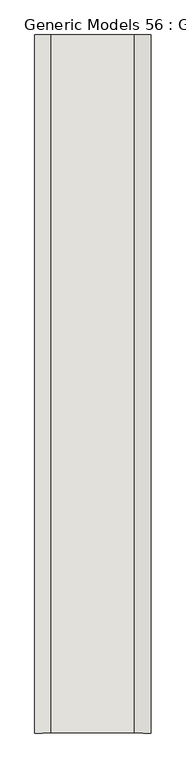
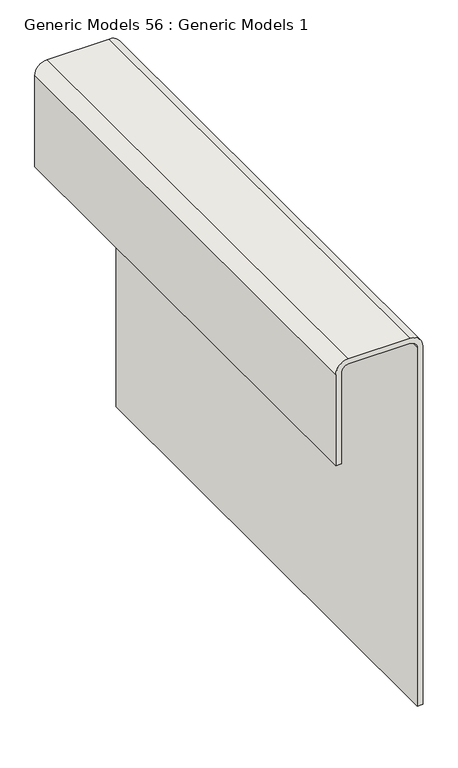
"""IFC4 building model written with IfcOpenShell, lengths in millimetres: wall geometry, Generic Models 56 : Generic Models 1."""

import ifcopenshell
import ifcopenshell.guid

model = None  # the IFC model being written
_history = None  # IfcOwnerHistory: only IFC2X3 demands one
_inside = {}  # id of a spatial element -> (the spatial element, [elements in it])
_under = {}  # id of a project, library or spatial element -> (it, [spatial elements below it])
_declared = {}  # id of a project -> (the project, [libraries it declares])
_typed = {}  # id of a type object -> (the type object, [elements of that type])
_made_of = {}  # id of a material, layer set ... -> (it, [elements and type objects made of it])


def new_model(schema):
    """Start an empty IFC model of exactly this schema.

    Asked for "IFC4X3", IfcOpenShell would pick the latest addendum, in which some entities
    have other attributes; the version numbers below select the first issue.
    IFC2X3 requires an IfcOwnerHistory on every rooted entity: one is made here for all.
    """
    global model, _history
    if schema == "IFC4X3":
        model = ifcopenshell.file(schema_version=(4, 3, 0, 0))
    else:
        model = ifcopenshell.file(schema=schema)
    _inside.clear()
    _under.clear()
    _declared.clear()
    _typed.clear()
    _made_of.clear()
    _history = None
    if model.schema == "IFC2X3":
        org = make("IfcOrganization", Name="unknown")
        user = make(
            "IfcPersonAndOrganization",
            ThePerson=make("IfcPerson", FamilyName="unknown"),
            TheOrganization=org,
        )
        app = make(
            "IfcApplication",
            ApplicationDeveloper=org,
            Version="unknown",
            ApplicationFullName="unknown",
            ApplicationIdentifier="unknown",
        )
        _history = make(
            "IfcOwnerHistory",
            OwningUser=user,
            OwningApplication=app,
            ChangeAction="ADDED",
            CreationDate=0,
        )
    return model


def make(cls, **values):
    """One entity of the class cls with the attributes given. An attribute that is None is left unset."""
    return model.create_entity(
        cls, **{name: value for name, value in values.items() if value is not None}
    )


def rooted(cls, **values):
    """An entity with a GlobalId (a new one), such as an element, a storey or a relation."""
    return make(cls, GlobalId=ifcopenshell.guid.new(), OwnerHistory=_history, **values)


def si_unit(unit_type, name, prefix=None):
    """IfcSIUnit, for example si_unit("LENGTHUNIT", "METRE", prefix="MILLI")."""
    return make("IfcSIUnit", UnitType=unit_type, Prefix=prefix, Name=name)


def assignment(units):
    """IfcUnitAssignment: the units of a project."""
    return None if units is None else make("IfcUnitAssignment", Units=units)


def point(xyz):
    """IfcCartesianPoint."""
    return None if xyz is None else make("IfcCartesianPoint", Coordinates=xyz)


def direction(xyz):
    """IfcDirection."""
    return None if xyz is None else make("IfcDirection", DirectionRatios=xyz)


def frame(location, z_axis=None, x_axis=None):
    """IfcAxis2Placement3D, a coordinate frame: its origin and axes. An axis left out is left unset."""
    return make(
        "IfcAxis2Placement3D",
        Location=point(location),
        Axis=direction(z_axis),
        RefDirection=direction(x_axis),
    )


def frame_2d(location, x_axis=None):
    """IfcAxis2Placement2D, a coordinate frame in the plane: its origin and x axis."""
    return make(
        "IfcAxis2Placement2D", Location=point(location), RefDirection=direction(x_axis)
    )


def origin():
    """The frame at (0, 0, 0) with its axes left unset."""
    return frame((0.0, 0.0, 0.0))


def place(relative_to, where):
    """IfcLocalPlacement: puts the frame where relative to a parent placement (None: the world)."""
    return make(
        "IfcLocalPlacement", PlacementRelTo=relative_to, RelativePlacement=where
    )


def context(
    kind, dimensions, precision=None, world=None, true_north=None, identifier=None
):
    """IfcGeometricRepresentationContext, for example the 3D "Model" context."""
    return make(
        "IfcGeometricRepresentationContext",
        ContextIdentifier=identifier,
        ContextType=kind,
        CoordinateSpaceDimension=dimensions,
        Precision=precision,
        WorldCoordinateSystem=world,
        TrueNorth=true_north,
    )


def project(units=None, contexts=None):
    """IfcProject with its units and contexts."""
    return rooted(
        "IfcProject",
        Name="project",
        RepresentationContexts=contexts,
        UnitsInContext=assignment(units),
    )


def spatial(cls, under=None, at=None, **own):
    """A site, building, storey or space (cls), placed at a placement, below another one or the project."""
    s = rooted(cls, ObjectPlacement=at, **own)
    if under is not None:
        _under.setdefault(under.id(), (under, []))[1].append(s)
    return s


def polyline(points):
    """IfcPolyline through the points."""
    return make("IfcPolyline", Points=[point(p) for p in points])


def circle_curve(where, radius):
    """IfcCircle in the frame where."""
    return make("IfcCircle", Position=where, Radius=radius)


def trimmed(basis, trim1, trim2, sense, master):
    """IfcTrimmedCurve: the piece of a basis curve between two trims."""
    return make(
        "IfcTrimmedCurve",
        BasisCurve=basis,
        Trim1=trim1,
        Trim2=trim2,
        SenseAgreement=sense,
        MasterRepresentation=master,
    )


def segment(curve, same_sense, transition):
    """IfcCompositeCurveSegment."""
    return make(
        "IfcCompositeCurveSegment",
        Transition=transition,
        SameSense=same_sense,
        ParentCurve=curve,
    )


def composite_curve(segments, self_intersect=None):
    """IfcCompositeCurve: segments joined end to end."""
    return make("IfcCompositeCurve", Segments=segments, SelfIntersect=self_intersect)


def outline(outer, holes=None, kind="AREA"):
    """IfcArbitraryClosedProfileDef: a profile drawn as a closed curve; with holes, ...WithVoids."""
    if holes is None:
        return make("IfcArbitraryClosedProfileDef", ProfileType=kind, OuterCurve=outer)
    return make(
        "IfcArbitraryProfileDefWithVoids",
        ProfileType=kind,
        OuterCurve=outer,
        InnerCurves=holes,
    )


def extrude(swept, where, along, depth):
    """IfcExtrudedAreaSolid: the profile swept, set in the frame where, extruded along a direction by depth."""
    return make(
        "IfcExtrudedAreaSolid",
        SweptArea=swept,
        Position=where,
        ExtrudedDirection=direction(along),
        Depth=depth,
    )


def shape(context_of_items, identifier, shape_type, items):
    """IfcShapeRepresentation: the items that make up one representation, for example the "Body"."""
    return make(
        "IfcShapeRepresentation",
        ContextOfItems=context_of_items,
        RepresentationIdentifier=identifier,
        RepresentationType=shape_type,
        Items=items,
    )


def source(mapping_origin, context_of_items, identifier, shape_type, items):
    """IfcRepresentationMap: a shape defined once, which mapped items show again and again."""
    return make(
        "IfcRepresentationMap",
        MappingOrigin=mapping_origin,
        MappedRepresentation=shape(context_of_items, identifier, shape_type, items),
    )


def transform(
    local_origin,
    x_axis=None,
    y_axis=None,
    z_axis=None,
    scale=None,
    scale2=None,
    scale3=None,
    uniform=True,
):
    """IfcCartesianTransformationOperator3D, or its non-uniform kind. x_axis, y_axis, z_axis: its Axis1, 2, 3."""
    if uniform:
        return make(
            "IfcCartesianTransformationOperator3D",
            Axis1=direction(x_axis),
            Axis2=direction(y_axis),
            LocalOrigin=point(local_origin),
            Scale=scale,
            Axis3=direction(z_axis),
        )
    return make(
        "IfcCartesianTransformationOperator3DnonUniform",
        Axis1=direction(x_axis),
        Axis2=direction(y_axis),
        LocalOrigin=point(local_origin),
        Scale=scale,
        Axis3=direction(z_axis),
        Scale2=scale2,
        Scale3=scale3,
    )


def mapped(mapping_source, mapping_target):
    """IfcMappedItem: shows the shape of a source again, moved by a transform."""
    return make(
        "IfcMappedItem", MappingSource=mapping_source, MappingTarget=mapping_target
    )


def made_of(thing, what):
    """Note that an element or type object is made of a material, layer set ...; save() writes the relation."""
    if what is not None:
        _made_of.setdefault(what.id(), (what, []))[1].append(thing)
    return thing


def element(
    cls,
    number,
    at=None,
    inside=None,
    cuts=None,
    type_object=None,
    material=None,
    context=None,
    identifier="Body",
    shape_type=None,
    held_by="IfcProductDefinitionShape",
    body=None,
    shapes=None,
    **own,
):
    """One element of the class cls, such as IfcWall. Its Tag is "e" and its number.

    at: its placement. inside: the storey or other place that contains it. cuts: it is an
    opening in that element (IfcRelVoidsElement). A single representation is given by context,
    identifier, shape_type and body (its items); several are given by shapes. held_by: the class
    of the entity that holds the representations. save() writes the other relations.
    """
    e = rooted(cls, Tag="e%d" % number, ObjectPlacement=at, **own)
    if body is not None:
        shapes = [shape(context, identifier, shape_type, body)]
    if shapes is not None:
        e.Representation = make(held_by, Representations=shapes)
    if inside is not None:
        _inside.setdefault(inside.id(), (inside, []))[1].append(e)
    if cuts is not None:
        rooted(
            "IfcRelVoidsElement", RelatingBuildingElement=cuts, RelatedOpeningElement=e
        )
    if type_object is not None:
        _typed.setdefault(type_object.id(), (type_object, []))[1].append(e)
    return made_of(e, material)


def aggregate(whole, parts):
    """IfcRelAggregates: a whole, such as a stair, and the parts it consists of."""
    return rooted("IfcRelAggregates", RelatingObject=whole, RelatedObjects=parts)


def save(model, path):
    """Write the relations noted so far, then the file.

    IfcRelAggregates (storeys below a building ...), IfcRelContainedInSpatialStructure (elements
    in a storey), IfcRelDefinesByType, IfcRelAssociatesMaterial and IfcRelDeclares: one each for
    every whole, place, type object, material and project.
    """
    for whole, parts in _under.values():
        aggregate(whole, parts)
    for where, things in _inside.values():
        rooted(
            "IfcRelContainedInSpatialStructure",
            RelatedElements=things,
            RelatingStructure=where,
        )
    for kind, things in _typed.values():
        rooted("IfcRelDefinesByType", RelatedObjects=things, RelatingType=kind)
    for what, things in _made_of.values():
        rooted("IfcRelAssociatesMaterial", RelatedObjects=things, RelatingMaterial=what)
    for by, libraries in _declared.values():
        rooted("IfcRelDeclares", RelatingContext=by, RelatedDefinitions=libraries)
    model.write(path)


def generic_models_56_generic_models_1_9cf2a8bd(model_context):
    return source(origin(), model_context, "Body", "SweptSolid", [
        extrude(outline(composite_curve([segment(polyline([(2136.4283305, 376659.775), (1251.002474, 376659.775), (1251.002474, 376672.475), (2136.4283305, 376672.475)]), True, "CONTINUOUS"), segment(trimmed(circle_curve(frame_2d((2136.4283305, 376643.5008565)), 28.9741435), [point((2136.4283305, 376672.475))], [point((2165.402474, 376643.5008565))], False, "CARTESIAN"), True, "CONTINUOUS"), segment(polyline([(2165.402474, 376643.5008565), (2165.402474, 376498.2491435)]), True, "CONTINUOUS"), segment(trimmed(circle_curve(frame_2d((2136.4283305, 376498.2491435)), 28.9741435), [point((2165.402474, 376498.2491435))], [point((2136.4283305, 376469.275))], False, "CARTESIAN"), True, "CONTINUOUS"), segment(polyline([(2136.4283305, 376469.275), (1911.402474, 376469.275), (1911.402474, 376481.975), (2136.4283305, 376481.975)]), True, "CONTINUOUS"), segment(trimmed(circle_curve(frame_2d((2136.4283305, 376498.2491435)), 16.2741435), [point((2136.4283305, 376481.975))], [point((2152.702474, 376498.2491435))], True, "CARTESIAN"), True, "CONTINUOUS"), segment(polyline([(2152.702474, 376498.2491435), (2152.702474, 376643.5008565)]), True, "CONTINUOUS"), segment(trimmed(circle_curve(frame_2d((2136.4283305, 376643.5008565)), 16.2741435), [point((2152.702474, 376643.5008565))], [point((2136.4283305, 376659.775))], True, "CARTESIAN"), True, "CONTINUOUS")], self_intersect=False)), frame((0.0, 76.2, 0.0), z_axis=(0.0, 1.0, 0.0), x_axis=(0.0, 0.0, 1.0)), (0.0, 0.0, 1.0), 1219.2),
    ])


if __name__ == "__main__":
    model = new_model("IFC4")
    model_context = context("Model", 3, world=origin())
    ifc_project = project(units=[si_unit("LENGTHUNIT", "METRE", prefix="MILLI")], contexts=[model_context])
    site = spatial("IfcSite", under=ifc_project)
    building = spatial("IfcBuilding", under=site)
    placement = place(None, origin())
    generic_models_56_generic_models_1_shape = generic_models_56_generic_models_1_9cf2a8bd(model_context)
    element("IfcWall", 1, ObjectType="Generic Models 56 : Generic Models 1", at=placement, inside=building, context=model_context, shape_type="MappedRepresentation", body=[
        mapped(generic_models_56_generic_models_1_shape, transform((0.0, 0.0, 0.0), x_axis=(1.0, 0.0, 0.0), y_axis=(0.0, 1.0, 0.0), z_axis=(0.0, 0.0, 1.0))),
    ])
    save(model, "model.ifc")

# Revit data of these elements
# Element 1 (IfcWall, "Generic Models 56 : Generic Models 1")
#   Materials on its faces: "WALL REINFORCING - SEE PLAN SCHEDULES FOR SIZE/LOCATION"
# Materials
#   "WALL REINFORCING - SEE PLAN SCHEDULES FOR SIZE/LOCATION": class "Metal", colour RGB 189 187 185, transparency 0, Description = "Structural steel 50ksi", Cost = 0
